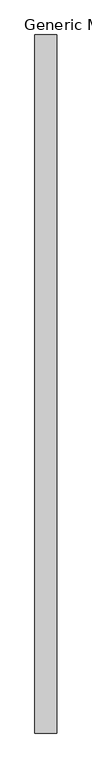
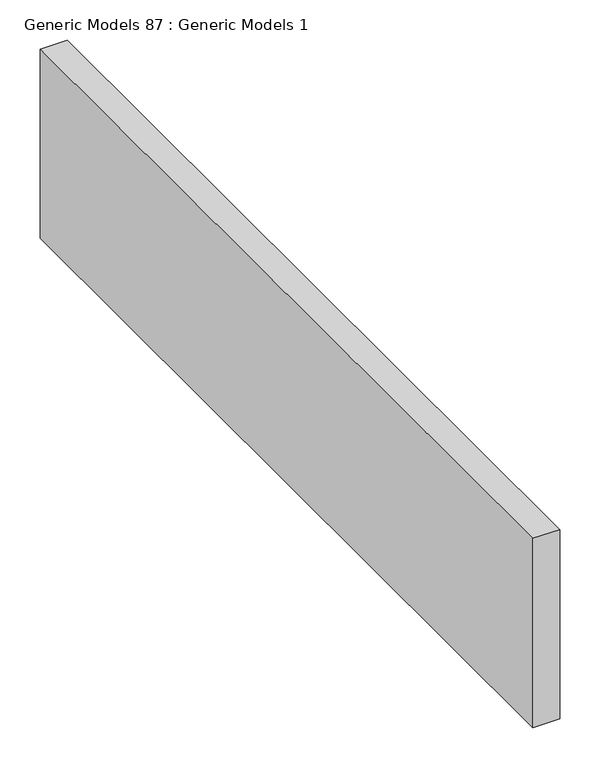
"""IFC4 building model written with IfcOpenShell, lengths in millimetres: proxy geometry, Generic Models 87 : Generic Models 1."""

from ifc_helpers import new_model, si_unit, frame, origin, place, context, project, spatial, polyline, outline, extrude, source, transform, mapped, element, save


def generic_models_87_generic_models_1_55a64953(model_context):
    return source(origin(), model_context, "Body", "SweptSolid", [
        extrude(outline(polyline([(51968.4, 0.0), (51930.3, 0.0), (51930.3, 1219.2), (51968.4, 1219.2), (51968.4, 0.0)])), frame((0.0, 0.0, 5222.478125), z_axis=(0.0, 0.0, 1.0), x_axis=(1.0, 0.0, 0.0)), (0.0, 0.0, 1.0), 285.75),
    ])


if __name__ == "__main__":
    model = new_model("IFC4")
    model_context = context("Model", 3, world=origin())
    ifc_project = project(units=[si_unit("LENGTHUNIT", "METRE", prefix="MILLI")], contexts=[model_context])
    site = spatial("IfcSite", under=ifc_project)
    building = spatial("IfcBuilding", under=site)
    placement = place(None, origin())
    generic_models_87_generic_models_1_shape = generic_models_87_generic_models_1_55a64953(model_context)
    element("IfcBuildingElementProxy", 1, Name="Generic Models 87 : Generic Models 1", ObjectType="Generic Models 87 : Generic Models 1", at=placement, inside=building, context=model_context, shape_type="MappedRepresentation", body=[
        mapped(generic_models_87_generic_models_1_shape, transform((0.0, 0.0, 0.0), x_axis=(1.0, 0.0, 0.0), y_axis=(0.0, 1.0, 0.0), z_axis=(0.0, 0.0, 1.0))),
    ])
    save(model, "model.ifc")

# Revit data of these elements
# Element 1 (IfcBuildingElementProxy, "Generic Models 87 : Generic Models 1")
#   Materials on its faces: "2X12 LEDGER WITH HILTI 3/8* DIAMETER HLC SLEEVE ANCHOR @ 8” OC."
# Materials
#   "2X12 LEDGER WITH HILTI 3/8* DIAMETER HLC SLEEVE ANCHOR @ 8” OC.": class "Wood", colour RGB 234 198 147, transparency 0, Description = "Pinus Echinata", Cost = 0
